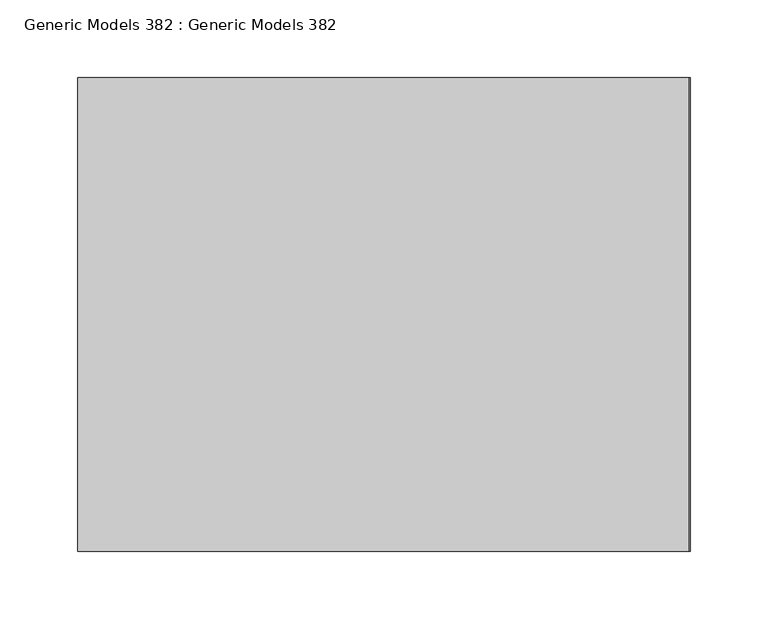
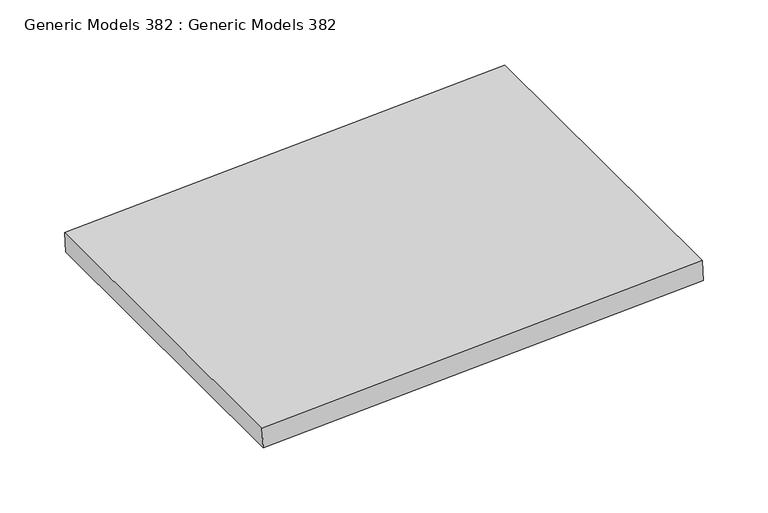
"""IFC4 building model written with IfcOpenShell, lengths in millimetres: proxy geometry, Generic Models 382 : Generic Models 382."""

from ifc_helpers import new_model, si_unit, frame, origin, place, context, project, spatial, polyline, outline, extrude, source, transform, mapped, element, save


def generic_models_382_generic_models_382_2764ce1a(model_context):
    return source(origin(), model_context, "Body", "SweptSolid", [
        extrude(outline(polyline([(0.0, -393.446218), (0.0, 0.0), (304.8, 0.0), (304.8, -393.446218), (0.0, -393.446218)])), frame((-7080.1562926, -4250.542257, 129127.2173365), z_axis=(-0.05233595624295883, 0.0, 0.9986295347545732), x_axis=(0.0, 1.0, 0.0)), (0.0, 0.0, 1.0), 19.05),
    ])


if __name__ == "__main__":
    model = new_model("IFC4")
    model_context = context("Model", 3, world=origin())
    ifc_project = project(units=[si_unit("LENGTHUNIT", "METRE", prefix="MILLI")], contexts=[model_context])
    site = spatial("IfcSite", under=ifc_project)
    building = spatial("IfcBuilding", under=site)
    placement = place(None, origin())
    generic_models_382_generic_models_382_shape = generic_models_382_generic_models_382_2764ce1a(model_context)
    element("IfcBuildingElementProxy", 1, Name="Generic Models 382 : Generic Models 382", ObjectType="Generic Models 382 : Generic Models 382", at=placement, inside=building, context=model_context, shape_type="MappedRepresentation", body=[
        mapped(generic_models_382_generic_models_382_shape, transform((0.0, 0.0, 0.0), x_axis=(1.0, 0.0, 0.0), y_axis=(0.0, 1.0, 0.0), z_axis=(0.0, 0.0, 1.0))),
    ])
    save(model, "model.ifc")

# Revit data of these elements
# Element 1 (IfcBuildingElementProxy, "Generic Models 382 : Generic Models 382")
#   Materials on its faces: "_CDX PLYWOOD -  SEE STRUCT DWGs"
# Materials
#   "_CDX PLYWOOD -  SEE STRUCT DWGs": class "Generic", colour RGB 98 75 74, transparency 0, Cost = 0
